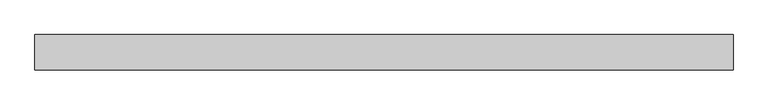
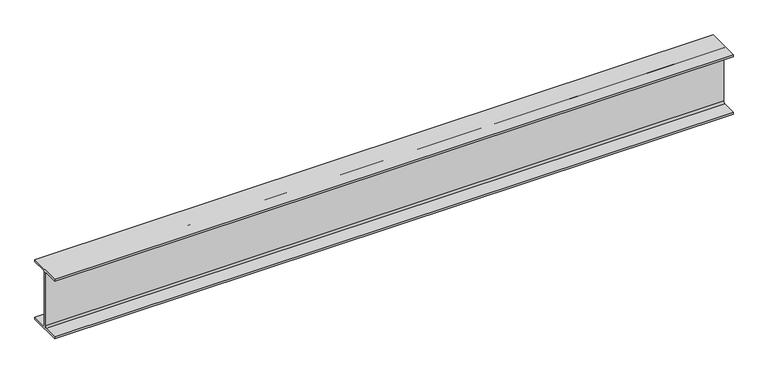
"""IFC4 building model written with IfcOpenShell, lengths in millimetres: beam geometry, Old_Steel Beam_H-KSD3502 : H_SB_ASB_H-200×200x8x12."""

from ifc_helpers import new_model, si_unit, point, frame, frame_2d, origin, place, context, project, spatial, polyline, circle_curve, trimmed, segment, composite_curve, outline, extrude, source, transform, mapped, element, save


def beam_deccd3ed(model_context):
    return source(origin(), model_context, "Body", "SweptSolid", [
        extrude(outline(composite_curve([segment(polyline([(82.5, -141.5), (82.5, -151.7), (-82.5, -151.7), (-82.5, -141.5), (-11.9, -141.5)]), True, "CONTINUOUS"), segment(trimmed(circle_curve(frame_2d((-11.9, -132.6)), 8.9), [point((-11.9, -141.5))], [point((-3.0, -132.6))], True, "CARTESIAN"), True, "CONTINUOUS"), segment(polyline([(-3.0, -132.6), (-3.0, 132.6)]), True, "CONTINUOUS"), segment(trimmed(circle_curve(frame_2d((-11.9, 132.6)), 8.9), [point((-3.0, 132.6))], [point((-11.9, 141.5))], True, "CARTESIAN"), True, "CONTINUOUS"), segment(polyline([(-11.9, 141.5), (-82.5, 141.5), (-82.5, 151.7), (82.5, 151.7), (82.5, 141.5), (11.9, 141.5)]), True, "CONTINUOUS"), segment(trimmed(circle_curve(frame_2d((11.9, 132.6)), 8.9), [point((11.9, 141.5))], [point((3.0, 132.6))], True, "CARTESIAN"), True, "CONTINUOUS"), segment(polyline([(3.0, 132.6), (3.0, -132.6)]), True, "CONTINUOUS"), segment(trimmed(circle_curve(frame_2d((11.9, -132.6)), 8.9), [point((3.0, -132.6))], [point((11.9, -141.5))], True, "CARTESIAN"), True, "CONTINUOUS"), segment(polyline([(11.9, -141.5), (82.5, -141.5)]), True, "CONTINUOUS")], self_intersect=False)), frame((-1686.0175372, 0.0, 0.0), z_axis=(1.0, 0.0, 0.0), x_axis=(0.0, 1.0, 0.0)), (0.0, 0.0, 1.0), 3267.7340685),
    ])


if __name__ == "__main__":
    model = new_model("IFC4")
    model_context = context("Model", 3, world=origin())
    ifc_project = project(units=[si_unit("LENGTHUNIT", "METRE", prefix="MILLI")], contexts=[model_context])
    site = spatial("IfcSite", under=ifc_project)
    building = spatial("IfcBuilding", under=site)
    placement = place(None, origin())
    beam_shape = beam_deccd3ed(model_context)
    element("IfcBeam", 1, ObjectType="Old_Steel Beam_H-KSD3502 : H_SB_ASB_H-200×200x8x12", at=placement, inside=building, context=model_context, shape_type="MappedRepresentation", body=[
        mapped(beam_shape, transform((0.0, 0.0, 0.0), x_axis=(1.0, 0.0, 0.0), y_axis=(0.0, 1.0, 0.0), z_axis=(0.0, 0.0, 1.0))),
    ])
    save(model, "model.ifc")

# Revit data of these elements
# Type "Old_Steel Beam_H-KSD3502 : H_SB_ASB_H-200×200x8x12"
#   Width = 20.0 cm
#   Web Thickness = 0.8 cm
#   Web Fillet = 1.3 cm
#   Warping Constant = 141376.0 cm⁶
#   Torsional Moment of Inertia = 26.2485 cm⁴
#   Torsional Modulus = 1.0 cm³
#   Section Area = 63.53 cm²
#   Plastic Modulus weak axis = 244.0 cm³
#   Plastic Modulus strong axis = 525.0 cm³
#   Perimeter = 1.16 m²/m
#   Nominal Weight = 49.90 kgf/m
#   Moment of Inertia weak axis = 1600.00 cm⁴
#   Moment of Inertia strong axis = 4720.00 cm⁴
#   Height = 20.0 cm
#   Flange Thickness = 1.2 cm
#   Elastic Modulus weak axis = 160.0 cm³
#   Elastic Modulus strong axis = 472.0 cm³
#   Centroid Vertical = 10.0 cm
#   Centroid Horizontal = 10.0 cm
#   Length [instance default] = 1.5240 m
#   Structural Material [instance default] = Steel, 45-345
#   Assembly Code = ""
# Element 1 (IfcBeam, "Old_Steel Beam_H-KSD3502 : H_SB_ASB_H-200×200x8x12")
#   Structural Material = none
# Materials
#   "Steel, 45-345": class "Metal", colour RGB 189 187 185, transparency 0, Description = "Steel 345 MPa", Cost = 0
